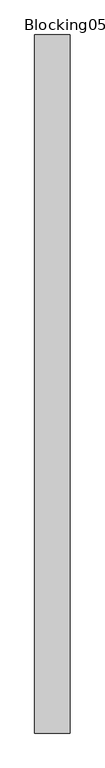
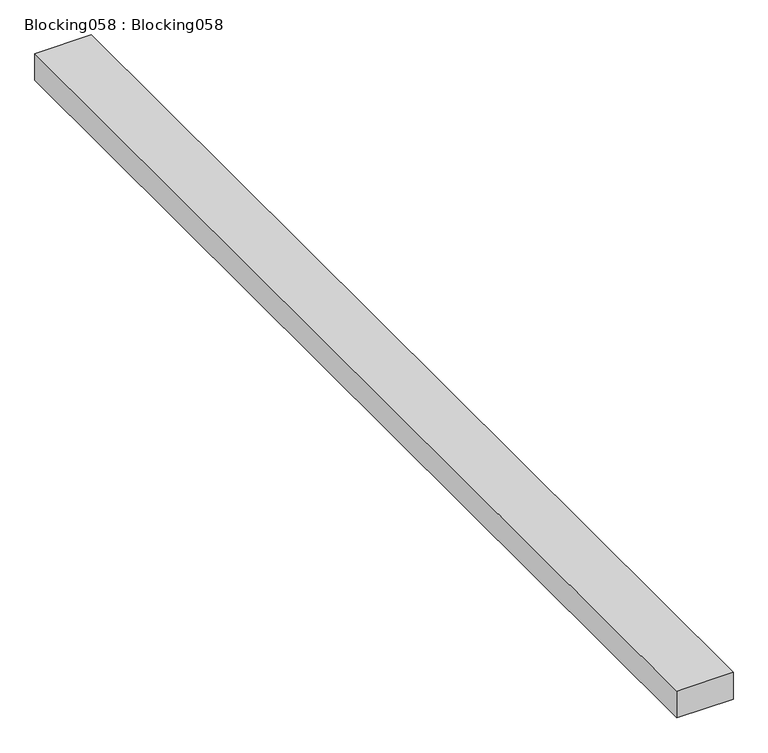
"""IFC4 building model written with IfcOpenShell, lengths in millimetres: proxy geometry, Blocking058 : Blocking058."""

from ifc_helpers import new_model, si_unit, frame, origin, place, context, project, spatial, polyline, outline, extrude, source, transform, mapped, element, save


def blocking058_blocking058_e5320c3e(model_context):
    return source(origin(), model_context, "Body", "SweptSolid", [
        extrude(outline(polyline([(-9298.3737014, 7982.1531721), (-9399.9737014, 7982.1531721), (-9399.9737014, 9982.1531721), (-9298.3737014, 9982.1531721), (-9298.3737014, 7982.1531721)])), frame((0.0, 0.0, 39953.9460083), z_axis=(0.0, 0.0, 1.0), x_axis=(1.0, 0.0, 0.0)), (0.0, 0.0, 1.0), 50.8),
    ])


if __name__ == "__main__":
    model = new_model("IFC4")
    model_context = context("Model", 3, world=origin())
    ifc_project = project(units=[si_unit("LENGTHUNIT", "METRE", prefix="MILLI")], contexts=[model_context])
    site = spatial("IfcSite", under=ifc_project)
    building = spatial("IfcBuilding", under=site)
    placement = place(None, origin())
    blocking058_blocking058_shape = blocking058_blocking058_e5320c3e(model_context)
    element("IfcBuildingElementProxy", 1, Name="Blocking058 : Blocking058", ObjectType="Blocking058 : Blocking058", at=placement, inside=building, context=model_context, shape_type="MappedRepresentation", body=[
        mapped(blocking058_blocking058_shape, transform((0.0, 0.0, 0.0), x_axis=(1.0, 0.0, 0.0), y_axis=(0.0, 1.0, 0.0), z_axis=(0.0, 0.0, 1.0))),
    ])
    save(model, "model.ifc")

# Revit data of these elements
# Type "Blocking058 : Blocking058"
#   NameOverride = "Blocking058"
# Element 1 (IfcBuildingElementProxy, "Blocking058 : Blocking058")
#   Materials on its faces: "WOOD BLOCKING AS REQUIRED"
# Materials
#   "WOOD BLOCKING AS REQUIRED": class "Unassigned", colour RGB 166 124 85, transparency 0, Cost = 0
